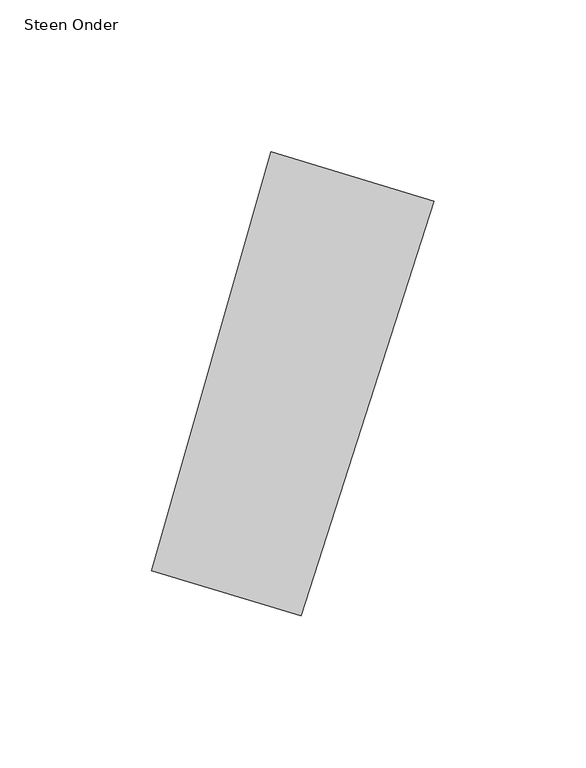
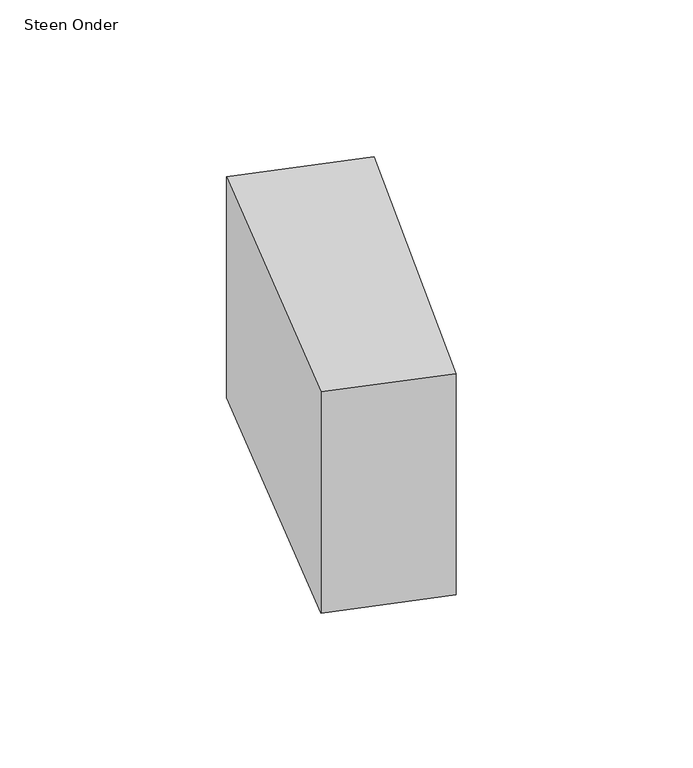
"""IFC4 building model written with IfcOpenShell, lengths in millimetres: proxy geometry, 00_GMA_steen_versie_4 : Steen Onder."""

from ifc_helpers import new_model, si_unit, origin, origin_with_axes, place, context, project, spatial, polyline, outline, extrude, source, transform, mapped, element, save


def steen_onder_3020a2e2(model_context):
    return source(origin(), model_context, "Body", "SweptSolid", [
        extrude(outline(polyline([(121.8746153, 135.9284681), (78.1631015, -0.508178), (29.0625992, 14.3301891), (68.2295243, 152.1402279), (121.8746153, 135.9284681)])), origin_with_axes(), (0.0, 0.0, 1.0), 100.0),
    ])


if __name__ == "__main__":
    model = new_model("IFC4")
    model_context = context("Model", 3, world=origin())
    ifc_project = project(units=[si_unit("LENGTHUNIT", "METRE", prefix="MILLI")], contexts=[model_context])
    site = spatial("IfcSite", under=ifc_project)
    building = spatial("IfcBuilding", under=site)
    placement = place(None, origin())
    steen_onder_shape = steen_onder_3020a2e2(model_context)
    element("IfcBuildingElementProxy", 1, Name="00_GMA_steen_versie_4 : Steen Onder", ObjectType="00_GMA_steen_versie_4 : Steen Onder", at=placement, inside=building, context=model_context, shape_type="MappedRepresentation", body=[
        mapped(steen_onder_shape, transform((0.0, 0.0, 0.0), x_axis=(1.0, 0.0, 0.0), y_axis=(0.0, 1.0, 0.0), z_axis=(0.0, 0.0, 1.0))),
    ])
    save(model, "model.ifc")

# Revit data of these elements
# Type "00_GMA_steen_versie_4 : Steen Onder"
#   StootVoegHalfBoven [instance default] = 5 mm
#   StootVoegHalf [instance default] = 5 mm
#   StootVoegBreedteOnder = 10 mm
#   StootVoegBreedteBoven = 10 mm
#   Steendikte = 100 mm
#   LintVoegOnderHalf = 0 mm
#   LintVoegOnder = 0 mm
#   LintVoegBovenHalf = 5 mm
#   LintVoegBoven = 10 mm
#   materiaal = none
#   MateriaalVoeg = none
#   Default Elevation = 0
